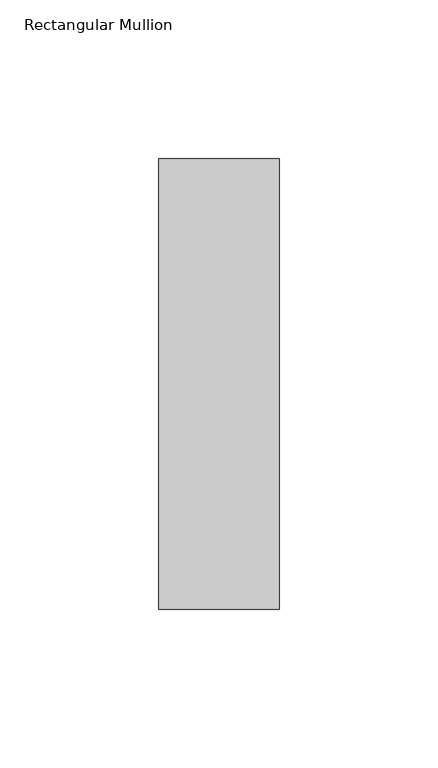
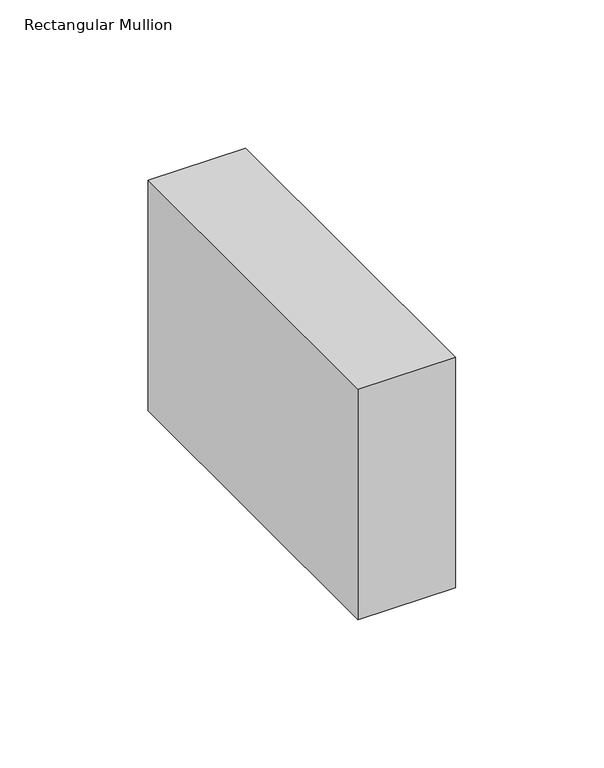
"""IFC4 building model written with IfcOpenShell, lengths in millimetres: member geometry, Rectangular Mullion : NLRS_21_CWM_hsb-regel 38x142_gen_rsf."""

from ifc_helpers import new_model, si_unit, frame, origin, place, context, project, spatial, polyline, outline, extrude, source, transform, mapped, element, save


def rectangular_mullion_d3b03aeb(model_context):
    return source(origin(), model_context, "Body", "SweptSolid", [
        extrude(outline(polyline([(0.0, -71.0), (-38.0, -71.0), (-38.0, 71.0), (0.0, 71.0), (0.0, -71.0)])), frame((0.0, 0.0, -94.9999997), z_axis=(0.0, 0.0, 1.0), x_axis=(1.0, 0.0, 0.0)), (0.0, 0.0, 1.0), 94.9999997),
    ])


if __name__ == "__main__":
    model = new_model("IFC4")
    model_context = context("Model", 3, world=origin())
    ifc_project = project(units=[si_unit("LENGTHUNIT", "METRE", prefix="MILLI")], contexts=[model_context])
    site = spatial("IfcSite", under=ifc_project)
    building = spatial("IfcBuilding", under=site)
    placement = place(None, origin())
    rectangular_mullion_shape = rectangular_mullion_d3b03aeb(model_context)
    element("IfcMember", 1, ObjectType="Rectangular Mullion : NLRS_21_CWM_hsb-regel 38x142_gen_rsf", at=placement, inside=building, context=model_context, shape_type="MappedRepresentation", body=[
        mapped(rectangular_mullion_shape, transform((0.0, 0.0, 0.0), x_axis=(1.0, 0.0, 0.0), y_axis=(0.0, 1.0, 0.0), z_axis=(0.0, 0.0, 1.0))),
    ])
    save(model, "model.ifc")

# Revit data of these elements
# Type "Rectangular Mullion : NLRS_21_CWM_hsb-regel 38x142_gen_rsf"
#   Export Type to IFC As = "IfcWall"
#   Type IfcGUID = "07M7mRoiH1CR8m_RSKIwpF"
#   Assembly Code = "21.10"
#   built-in parameter 1007322 = 0.465879 (stored number, unit not read)
#   built-in parameter 1007321 = 0.062336 (stored number, unit not read)
#   built-in parameter 1007320 = 0.062336 (stored number, unit not read)
# Element 1 (IfcMember, "Rectangular Mullion : NLRS_21_CWM_hsb-regel 38x142_gen_rsf")
#   Materials on its faces: "NLRS_i2_hout naaldhout vuren_gen_rsf"
# Materials
#   "NLRS_i2_hout naaldhout vuren_gen_rsf": class "I - Hout", colour RGB 234 199 147, transparency 0, Keynote = "i2", Manufacturer = "Revit Standards Foundation", URL = "www.revitstandards.org", Description = "hout vuren", Cost = 0
